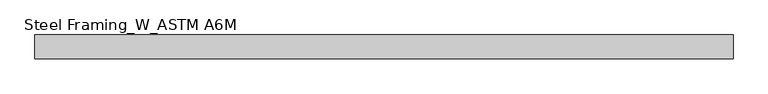
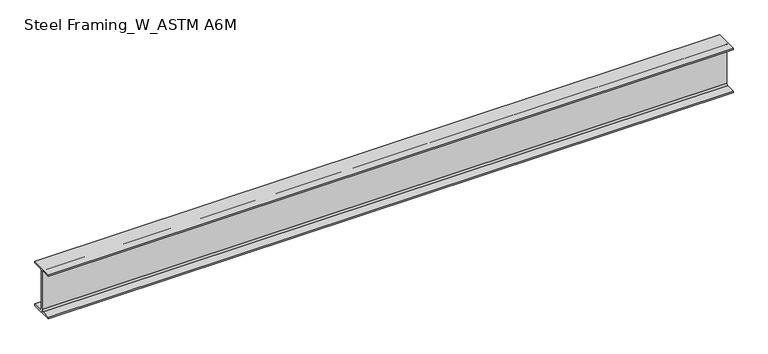
"""IFC4 building model written with IfcOpenShell, lengths in millimetres: beam geometry, Steel Framing_W_ASTM A6M : H_SB_AR_S02_W200x22.5_RB5."""

from ifc_helpers import new_model, si_unit, point, frame, frame_2d, origin, place, context, project, spatial, polyline, circle_curve, trimmed, segment, composite_curve, outline, extrude, source, transform, mapped, element, save


def steel_framing_w_astm_a6m_902f7afb(model_context):
    return source(origin(), model_context, "Body", "SweptSolid", [
        extrude(outline(composite_curve([segment(polyline([(51.0, -95.0), (51.0, -103.0), (-51.0, -103.0), (-51.0, -95.0), (-10.71, -95.0)]), True, "CONTINUOUS"), segment(trimmed(circle_curve(frame_2d((-10.71, -87.4)), 7.6), [point((-10.71, -95.0))], [point((-3.11, -87.4))], True, "CARTESIAN"), True, "CONTINUOUS"), segment(polyline([(-3.11, -87.4), (-3.11, 87.4)]), True, "CONTINUOUS"), segment(trimmed(circle_curve(frame_2d((-10.71, 87.4)), 7.6), [point((-3.11, 87.4))], [point((-10.71, 95.0))], True, "CARTESIAN"), True, "CONTINUOUS"), segment(polyline([(-10.71, 95.0), (-51.0, 95.0), (-51.0, 103.0), (51.0, 103.0), (51.0, 95.0), (10.71, 95.0)]), True, "CONTINUOUS"), segment(trimmed(circle_curve(frame_2d((10.71, 87.4)), 7.6), [point((10.71, 95.0))], [point((3.11, 87.4))], True, "CARTESIAN"), True, "CONTINUOUS"), segment(polyline([(3.11, 87.4), (3.11, -87.4)]), True, "CONTINUOUS"), segment(trimmed(circle_curve(frame_2d((10.71, -87.4)), 7.6), [point((3.11, -87.4))], [point((10.71, -95.0))], True, "CARTESIAN"), True, "CONTINUOUS"), segment(polyline([(10.71, -95.0), (51.0, -95.0)]), True, "CONTINUOUS")], self_intersect=False)), frame((-1500.0, 0.0, 0.0), z_axis=(1.0, 0.0, 0.0), x_axis=(0.0, 1.0, 0.0)), (0.0, 0.0, 1.0), 3000.0),
    ])


if __name__ == "__main__":
    model = new_model("IFC4")
    model_context = context("Model", 3, world=origin())
    ifc_project = project(units=[si_unit("LENGTHUNIT", "METRE", prefix="MILLI")], contexts=[model_context])
    site = spatial("IfcSite", under=ifc_project)
    building = spatial("IfcBuilding", under=site)
    placement = place(None, origin())
    steel_framing_w_astm_a6m_shape = steel_framing_w_astm_a6m_902f7afb(model_context)
    element("IfcBeam", 1, ObjectType="Steel Framing_W_ASTM A6M : H_SB_AR_S02_W200x22.5_RB5", at=placement, inside=building, context=model_context, shape_type="MappedRepresentation", body=[
        mapped(steel_framing_w_astm_a6m_shape, transform((0.0, 0.0, 0.0), x_axis=(1.0, 0.0, 0.0), y_axis=(0.0, 1.0, 0.0), z_axis=(0.0, 0.0, 1.0))),
    ])
    save(model, "model.ifc")

# Revit data of these elements
# Type "Steel Framing_W_ASTM A6M : H_SB_AR_S02_W200x22.5_RB5"
#   Type Mark = "RB5"
#   Section Name Key = "W8x15"
#   Width = 10.2 cm
#   Web Thickness = 0.622 cm
#   Web Fillet = 0.76 cm
#   Warping Constant = 13900.0 cm⁶
#   Torsional Moment of Inertia = 5.70 cm⁴
#   Section Area = 28.6 cm²
#   Plastic Modulus weak axis = 43.8 cm³
#   Plastic Modulus strong axis = 223.0 cm³
#   Perimeter = 0.795 m²/m
#   Nominal Weight = 22.50 kgf/m
#   Moment of Inertia weak axis = 142.00 cm⁴
#   Moment of Inertia strong axis = 2000.00 cm⁴
#   Height = 20.6 cm
#   Flange Thickness = 0.8 cm
#   Elastic Modulus weak axis = 27.9 cm³
#   Elastic Modulus strong axis = 193.0 cm³
#   Centroid Vertical = 10.3 cm
#   Centroid Horizontal = 5.1 cm
#   Length [instance default] = 1500 mm
#   Structural Material [instance default] = Steel, 45-345
#   Bolt Spacing = 0
#   Assembly Code = ""
# Element 1 (IfcBeam, "Steel Framing_W_ASTM A6M : H_SB_AR_S02_W200x22.5_RB5")
#   Materials on its faces: "Steel, 45-345"
# Materials
#   "Steel, 45-345": class "Metal", colour RGB 189 187 185, transparency 0, Description = "Steel 345 MPa", Cost = 0
